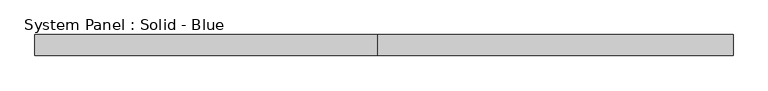
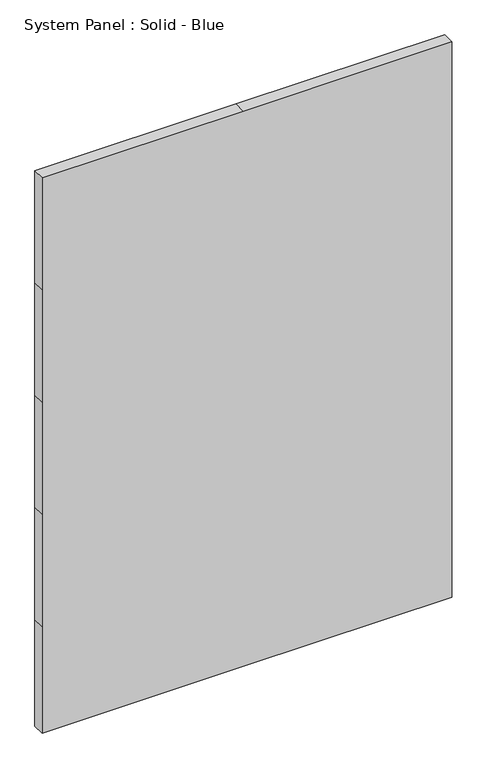
"""IFC4 building model written with IfcOpenShell, lengths in millimetres: plate geometry, System Panel : Solid - Blue."""

import ifcopenshell
import ifcopenshell.guid

model = None  # the IFC model being written
_history = None  # IfcOwnerHistory: only IFC2X3 demands one
_inside = {}  # id of a spatial element -> (the spatial element, [elements in it])
_under = {}  # id of a project, library or spatial element -> (it, [spatial elements below it])
_declared = {}  # id of a project -> (the project, [libraries it declares])
_typed = {}  # id of a type object -> (the type object, [elements of that type])
_made_of = {}  # id of a material, layer set ... -> (it, [elements and type objects made of it])


def new_model(schema):
    """Start an empty IFC model of exactly this schema.

    Asked for "IFC4X3", IfcOpenShell would pick the latest addendum, in which some entities
    have other attributes; the version numbers below select the first issue.
    IFC2X3 requires an IfcOwnerHistory on every rooted entity: one is made here for all.
    """
    global model, _history
    if schema == "IFC4X3":
        model = ifcopenshell.file(schema_version=(4, 3, 0, 0))
    else:
        model = ifcopenshell.file(schema=schema)
    _inside.clear()
    _under.clear()
    _declared.clear()
    _typed.clear()
    _made_of.clear()
    _history = None
    if model.schema == "IFC2X3":
        org = make("IfcOrganization", Name="unknown")
        user = make(
            "IfcPersonAndOrganization",
            ThePerson=make("IfcPerson", FamilyName="unknown"),
            TheOrganization=org,
        )
        app = make(
            "IfcApplication",
            ApplicationDeveloper=org,
            Version="unknown",
            ApplicationFullName="unknown",
            ApplicationIdentifier="unknown",
        )
        _history = make(
            "IfcOwnerHistory",
            OwningUser=user,
            OwningApplication=app,
            ChangeAction="ADDED",
            CreationDate=0,
        )
    return model


def make(cls, **values):
    """One entity of the class cls with the attributes given. An attribute that is None is left unset."""
    return model.create_entity(
        cls, **{name: value for name, value in values.items() if value is not None}
    )


def rooted(cls, **values):
    """An entity with a GlobalId (a new one), such as an element, a storey or a relation."""
    return make(cls, GlobalId=ifcopenshell.guid.new(), OwnerHistory=_history, **values)


def si_unit(unit_type, name, prefix=None):
    """IfcSIUnit, for example si_unit("LENGTHUNIT", "METRE", prefix="MILLI")."""
    return make("IfcSIUnit", UnitType=unit_type, Prefix=prefix, Name=name)


def assignment(units):
    """IfcUnitAssignment: the units of a project."""
    return None if units is None else make("IfcUnitAssignment", Units=units)


def point(xyz):
    """IfcCartesianPoint."""
    return None if xyz is None else make("IfcCartesianPoint", Coordinates=xyz)


def direction(xyz):
    """IfcDirection."""
    return None if xyz is None else make("IfcDirection", DirectionRatios=xyz)


def frame(location, z_axis=None, x_axis=None):
    """IfcAxis2Placement3D, a coordinate frame: its origin and axes. An axis left out is left unset."""
    return make(
        "IfcAxis2Placement3D",
        Location=point(location),
        Axis=direction(z_axis),
        RefDirection=direction(x_axis),
    )


def origin():
    """The frame at (0, 0, 0) with its axes left unset."""
    return frame((0.0, 0.0, 0.0))


def place(relative_to, where):
    """IfcLocalPlacement: puts the frame where relative to a parent placement (None: the world)."""
    return make(
        "IfcLocalPlacement", PlacementRelTo=relative_to, RelativePlacement=where
    )


def context(
    kind, dimensions, precision=None, world=None, true_north=None, identifier=None
):
    """IfcGeometricRepresentationContext, for example the 3D "Model" context."""
    return make(
        "IfcGeometricRepresentationContext",
        ContextIdentifier=identifier,
        ContextType=kind,
        CoordinateSpaceDimension=dimensions,
        Precision=precision,
        WorldCoordinateSystem=world,
        TrueNorth=true_north,
    )


def project(units=None, contexts=None):
    """IfcProject with its units and contexts."""
    return rooted(
        "IfcProject",
        Name="project",
        RepresentationContexts=contexts,
        UnitsInContext=assignment(units),
    )


def spatial(cls, under=None, at=None, **own):
    """A site, building, storey or space (cls), placed at a placement, below another one or the project."""
    s = rooted(cls, ObjectPlacement=at, **own)
    if under is not None:
        _under.setdefault(under.id(), (under, []))[1].append(s)
    return s


def polyline(points):
    """IfcPolyline through the points."""
    return make("IfcPolyline", Points=[point(p) for p in points])


def outline(outer, holes=None, kind="AREA"):
    """IfcArbitraryClosedProfileDef: a profile drawn as a closed curve; with holes, ...WithVoids."""
    if holes is None:
        return make("IfcArbitraryClosedProfileDef", ProfileType=kind, OuterCurve=outer)
    return make(
        "IfcArbitraryProfileDefWithVoids",
        ProfileType=kind,
        OuterCurve=outer,
        InnerCurves=holes,
    )


def extrude(swept, where, along, depth):
    """IfcExtrudedAreaSolid: the profile swept, set in the frame where, extruded along a direction by depth."""
    return make(
        "IfcExtrudedAreaSolid",
        SweptArea=swept,
        Position=where,
        ExtrudedDirection=direction(along),
        Depth=depth,
    )


def shape(context_of_items, identifier, shape_type, items):
    """IfcShapeRepresentation: the items that make up one representation, for example the "Body"."""
    return make(
        "IfcShapeRepresentation",
        ContextOfItems=context_of_items,
        RepresentationIdentifier=identifier,
        RepresentationType=shape_type,
        Items=items,
    )


def source(mapping_origin, context_of_items, identifier, shape_type, items):
    """IfcRepresentationMap: a shape defined once, which mapped items show again and again."""
    return make(
        "IfcRepresentationMap",
        MappingOrigin=mapping_origin,
        MappedRepresentation=shape(context_of_items, identifier, shape_type, items),
    )


def transform(
    local_origin,
    x_axis=None,
    y_axis=None,
    z_axis=None,
    scale=None,
    scale2=None,
    scale3=None,
    uniform=True,
):
    """IfcCartesianTransformationOperator3D, or its non-uniform kind. x_axis, y_axis, z_axis: its Axis1, 2, 3."""
    if uniform:
        return make(
            "IfcCartesianTransformationOperator3D",
            Axis1=direction(x_axis),
            Axis2=direction(y_axis),
            LocalOrigin=point(local_origin),
            Scale=scale,
            Axis3=direction(z_axis),
        )
    return make(
        "IfcCartesianTransformationOperator3DnonUniform",
        Axis1=direction(x_axis),
        Axis2=direction(y_axis),
        LocalOrigin=point(local_origin),
        Scale=scale,
        Axis3=direction(z_axis),
        Scale2=scale2,
        Scale3=scale3,
    )


def mapped(mapping_source, mapping_target):
    """IfcMappedItem: shows the shape of a source again, moved by a transform."""
    return make(
        "IfcMappedItem", MappingSource=mapping_source, MappingTarget=mapping_target
    )


def made_of(thing, what):
    """Note that an element or type object is made of a material, layer set ...; save() writes the relation."""
    if what is not None:
        _made_of.setdefault(what.id(), (what, []))[1].append(thing)
    return thing


def element(
    cls,
    number,
    at=None,
    inside=None,
    cuts=None,
    type_object=None,
    material=None,
    context=None,
    identifier="Body",
    shape_type=None,
    held_by="IfcProductDefinitionShape",
    body=None,
    shapes=None,
    **own,
):
    """One element of the class cls, such as IfcWall. Its Tag is "e" and its number.

    at: its placement. inside: the storey or other place that contains it. cuts: it is an
    opening in that element (IfcRelVoidsElement). A single representation is given by context,
    identifier, shape_type and body (its items); several are given by shapes. held_by: the class
    of the entity that holds the representations. save() writes the other relations.
    """
    e = rooted(cls, Tag="e%d" % number, ObjectPlacement=at, **own)
    if body is not None:
        shapes = [shape(context, identifier, shape_type, body)]
    if shapes is not None:
        e.Representation = make(held_by, Representations=shapes)
    if inside is not None:
        _inside.setdefault(inside.id(), (inside, []))[1].append(e)
    if cuts is not None:
        rooted(
            "IfcRelVoidsElement", RelatingBuildingElement=cuts, RelatedOpeningElement=e
        )
    if type_object is not None:
        _typed.setdefault(type_object.id(), (type_object, []))[1].append(e)
    return made_of(e, material)


def aggregate(whole, parts):
    """IfcRelAggregates: a whole, such as a stair, and the parts it consists of."""
    return rooted("IfcRelAggregates", RelatingObject=whole, RelatedObjects=parts)


def save(model, path):
    """Write the relations noted so far, then the file.

    IfcRelAggregates (storeys below a building ...), IfcRelContainedInSpatialStructure (elements
    in a storey), IfcRelDefinesByType, IfcRelAssociatesMaterial and IfcRelDeclares: one each for
    every whole, place, type object, material and project.
    """
    for whole, parts in _under.values():
        aggregate(whole, parts)
    for where, things in _inside.values():
        rooted(
            "IfcRelContainedInSpatialStructure",
            RelatedElements=things,
            RelatingStructure=where,
        )
    for kind, things in _typed.values():
        rooted("IfcRelDefinesByType", RelatedObjects=things, RelatingType=kind)
    for what, things in _made_of.values():
        rooted("IfcRelAssociatesMaterial", RelatedObjects=things, RelatingMaterial=what)
    for by, libraries in _declared.values():
        rooted("IfcRelDeclares", RelatingContext=by, RelatedDefinitions=libraries)
    model.write(path)


def system_panel_solid_blue_87c3cd20(model_context):
    return source(origin(), model_context, "Body", "SweptSolid", [
        extrude(outline(polyline([(0.0, -1052.2857143), (0.0, -18.1428571), (0.0, 1052.2857143), (577.85, 1052.2857143), (1187.45, 1052.2857143), (1797.05, 1052.2857143), (2406.65, 1052.2857143), (3016.25, 1052.2857143), (3016.25, -18.1428571), (3016.25, -1052.2857143), (2406.65, -1052.2857143), (1797.05, -1052.2857143), (1187.45, -1052.2857143), (577.85, -1052.2857143), (0.0, -1052.2857143)])), frame((0.0, -19.05, 0.0), z_axis=(0.0, 1.0, 0.0), x_axis=(0.0, 0.0, 1.0)), (0.0, 0.0, 1.0), 63.5),
    ])


if __name__ == "__main__":
    model = new_model("IFC4")
    model_context = context("Model", 3, world=origin())
    ifc_project = project(units=[si_unit("LENGTHUNIT", "METRE", prefix="MILLI")], contexts=[model_context])
    site = spatial("IfcSite", under=ifc_project)
    building = spatial("IfcBuilding", under=site)
    placement = place(None, origin())
    system_panel_solid_blue_shape = system_panel_solid_blue_87c3cd20(model_context)
    element("IfcPlate", 1, ObjectType="System Panel : Solid - Blue", at=placement, inside=building, context=model_context, shape_type="MappedRepresentation", body=[
        mapped(system_panel_solid_blue_shape, transform((0.0, 0.0, 0.0), x_axis=(1.0, 0.0, 0.0), y_axis=(0.0, 1.0, 0.0), z_axis=(0.0, 0.0, 1.0))),
    ])
    save(model, "model.ifc")

# Revit data of these elements
# Element 1 (IfcPlate, "System Panel : Solid - Blue")
#   Materials on its faces: "Blue Panel"
# Materials
#   "Blue Panel": class "Unassigned", colour RGB 0 0 160, transparency 0
